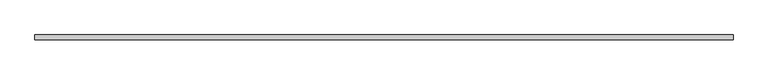
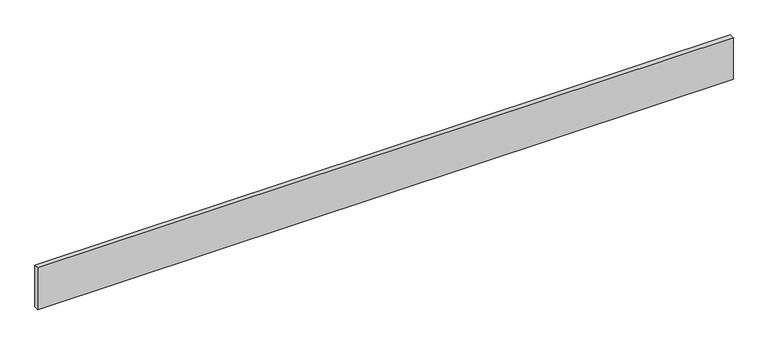
"""IFC4 building model written with IfcOpenShell, lengths in millimetres: proxy geometry, Joint001 1294 : Joint001 1294."""

import ifcopenshell
import ifcopenshell.guid

model = None  # the IFC model being written
_history = None  # IfcOwnerHistory: only IFC2X3 demands one
_inside = {}  # id of a spatial element -> (the spatial element, [elements in it])
_under = {}  # id of a project, library or spatial element -> (it, [spatial elements below it])
_declared = {}  # id of a project -> (the project, [libraries it declares])
_typed = {}  # id of a type object -> (the type object, [elements of that type])
_made_of = {}  # id of a material, layer set ... -> (it, [elements and type objects made of it])


def new_model(schema):
    """Start an empty IFC model of exactly this schema.

    Asked for "IFC4X3", IfcOpenShell would pick the latest addendum, in which some entities
    have other attributes; the version numbers below select the first issue.
    IFC2X3 requires an IfcOwnerHistory on every rooted entity: one is made here for all.
    """
    global model, _history
    if schema == "IFC4X3":
        model = ifcopenshell.file(schema_version=(4, 3, 0, 0))
    else:
        model = ifcopenshell.file(schema=schema)
    _inside.clear()
    _under.clear()
    _declared.clear()
    _typed.clear()
    _made_of.clear()
    _history = None
    if model.schema == "IFC2X3":
        org = make("IfcOrganization", Name="unknown")
        user = make(
            "IfcPersonAndOrganization",
            ThePerson=make("IfcPerson", FamilyName="unknown"),
            TheOrganization=org,
        )
        app = make(
            "IfcApplication",
            ApplicationDeveloper=org,
            Version="unknown",
            ApplicationFullName="unknown",
            ApplicationIdentifier="unknown",
        )
        _history = make(
            "IfcOwnerHistory",
            OwningUser=user,
            OwningApplication=app,
            ChangeAction="ADDED",
            CreationDate=0,
        )
    return model


def make(cls, **values):
    """One entity of the class cls with the attributes given. An attribute that is None is left unset."""
    return model.create_entity(
        cls, **{name: value for name, value in values.items() if value is not None}
    )


def rooted(cls, **values):
    """An entity with a GlobalId (a new one), such as an element, a storey or a relation."""
    return make(cls, GlobalId=ifcopenshell.guid.new(), OwnerHistory=_history, **values)


def si_unit(unit_type, name, prefix=None):
    """IfcSIUnit, for example si_unit("LENGTHUNIT", "METRE", prefix="MILLI")."""
    return make("IfcSIUnit", UnitType=unit_type, Prefix=prefix, Name=name)


def assignment(units):
    """IfcUnitAssignment: the units of a project."""
    return None if units is None else make("IfcUnitAssignment", Units=units)


def point(xyz):
    """IfcCartesianPoint."""
    return None if xyz is None else make("IfcCartesianPoint", Coordinates=xyz)


def direction(xyz):
    """IfcDirection."""
    return None if xyz is None else make("IfcDirection", DirectionRatios=xyz)


def frame(location, z_axis=None, x_axis=None):
    """IfcAxis2Placement3D, a coordinate frame: its origin and axes. An axis left out is left unset."""
    return make(
        "IfcAxis2Placement3D",
        Location=point(location),
        Axis=direction(z_axis),
        RefDirection=direction(x_axis),
    )


def origin():
    """The frame at (0, 0, 0) with its axes left unset."""
    return frame((0.0, 0.0, 0.0))


def place(relative_to, where):
    """IfcLocalPlacement: puts the frame where relative to a parent placement (None: the world)."""
    return make(
        "IfcLocalPlacement", PlacementRelTo=relative_to, RelativePlacement=where
    )


def context(
    kind, dimensions, precision=None, world=None, true_north=None, identifier=None
):
    """IfcGeometricRepresentationContext, for example the 3D "Model" context."""
    return make(
        "IfcGeometricRepresentationContext",
        ContextIdentifier=identifier,
        ContextType=kind,
        CoordinateSpaceDimension=dimensions,
        Precision=precision,
        WorldCoordinateSystem=world,
        TrueNorth=true_north,
    )


def project(units=None, contexts=None):
    """IfcProject with its units and contexts."""
    return rooted(
        "IfcProject",
        Name="project",
        RepresentationContexts=contexts,
        UnitsInContext=assignment(units),
    )


def spatial(cls, under=None, at=None, **own):
    """A site, building, storey or space (cls), placed at a placement, below another one or the project."""
    s = rooted(cls, ObjectPlacement=at, **own)
    if under is not None:
        _under.setdefault(under.id(), (under, []))[1].append(s)
    return s


def polyline(points):
    """IfcPolyline through the points."""
    return make("IfcPolyline", Points=[point(p) for p in points])


def outline(outer, holes=None, kind="AREA"):
    """IfcArbitraryClosedProfileDef: a profile drawn as a closed curve; with holes, ...WithVoids."""
    if holes is None:
        return make("IfcArbitraryClosedProfileDef", ProfileType=kind, OuterCurve=outer)
    return make(
        "IfcArbitraryProfileDefWithVoids",
        ProfileType=kind,
        OuterCurve=outer,
        InnerCurves=holes,
    )


def extrude(swept, where, along, depth):
    """IfcExtrudedAreaSolid: the profile swept, set in the frame where, extruded along a direction by depth."""
    return make(
        "IfcExtrudedAreaSolid",
        SweptArea=swept,
        Position=where,
        ExtrudedDirection=direction(along),
        Depth=depth,
    )


def shape(context_of_items, identifier, shape_type, items):
    """IfcShapeRepresentation: the items that make up one representation, for example the "Body"."""
    return make(
        "IfcShapeRepresentation",
        ContextOfItems=context_of_items,
        RepresentationIdentifier=identifier,
        RepresentationType=shape_type,
        Items=items,
    )


def source(mapping_origin, context_of_items, identifier, shape_type, items):
    """IfcRepresentationMap: a shape defined once, which mapped items show again and again."""
    return make(
        "IfcRepresentationMap",
        MappingOrigin=mapping_origin,
        MappedRepresentation=shape(context_of_items, identifier, shape_type, items),
    )


def transform(
    local_origin,
    x_axis=None,
    y_axis=None,
    z_axis=None,
    scale=None,
    scale2=None,
    scale3=None,
    uniform=True,
):
    """IfcCartesianTransformationOperator3D, or its non-uniform kind. x_axis, y_axis, z_axis: its Axis1, 2, 3."""
    if uniform:
        return make(
            "IfcCartesianTransformationOperator3D",
            Axis1=direction(x_axis),
            Axis2=direction(y_axis),
            LocalOrigin=point(local_origin),
            Scale=scale,
            Axis3=direction(z_axis),
        )
    return make(
        "IfcCartesianTransformationOperator3DnonUniform",
        Axis1=direction(x_axis),
        Axis2=direction(y_axis),
        LocalOrigin=point(local_origin),
        Scale=scale,
        Axis3=direction(z_axis),
        Scale2=scale2,
        Scale3=scale3,
    )


def mapped(mapping_source, mapping_target):
    """IfcMappedItem: shows the shape of a source again, moved by a transform."""
    return make(
        "IfcMappedItem", MappingSource=mapping_source, MappingTarget=mapping_target
    )


def made_of(thing, what):
    """Note that an element or type object is made of a material, layer set ...; save() writes the relation."""
    if what is not None:
        _made_of.setdefault(what.id(), (what, []))[1].append(thing)
    return thing


def element(
    cls,
    number,
    at=None,
    inside=None,
    cuts=None,
    type_object=None,
    material=None,
    context=None,
    identifier="Body",
    shape_type=None,
    held_by="IfcProductDefinitionShape",
    body=None,
    shapes=None,
    **own,
):
    """One element of the class cls, such as IfcWall. Its Tag is "e" and its number.

    at: its placement. inside: the storey or other place that contains it. cuts: it is an
    opening in that element (IfcRelVoidsElement). A single representation is given by context,
    identifier, shape_type and body (its items); several are given by shapes. held_by: the class
    of the entity that holds the representations. save() writes the other relations.
    """
    e = rooted(cls, Tag="e%d" % number, ObjectPlacement=at, **own)
    if body is not None:
        shapes = [shape(context, identifier, shape_type, body)]
    if shapes is not None:
        e.Representation = make(held_by, Representations=shapes)
    if inside is not None:
        _inside.setdefault(inside.id(), (inside, []))[1].append(e)
    if cuts is not None:
        rooted(
            "IfcRelVoidsElement", RelatingBuildingElement=cuts, RelatedOpeningElement=e
        )
    if type_object is not None:
        _typed.setdefault(type_object.id(), (type_object, []))[1].append(e)
    return made_of(e, material)


def aggregate(whole, parts):
    """IfcRelAggregates: a whole, such as a stair, and the parts it consists of."""
    return rooted("IfcRelAggregates", RelatingObject=whole, RelatedObjects=parts)


def save(model, path):
    """Write the relations noted so far, then the file.

    IfcRelAggregates (storeys below a building ...), IfcRelContainedInSpatialStructure (elements
    in a storey), IfcRelDefinesByType, IfcRelAssociatesMaterial and IfcRelDeclares: one each for
    every whole, place, type object, material and project.
    """
    for whole, parts in _under.values():
        aggregate(whole, parts)
    for where, things in _inside.values():
        rooted(
            "IfcRelContainedInSpatialStructure",
            RelatedElements=things,
            RelatingStructure=where,
        )
    for kind, things in _typed.values():
        rooted("IfcRelDefinesByType", RelatedObjects=things, RelatingType=kind)
    for what, things in _made_of.values():
        rooted("IfcRelAssociatesMaterial", RelatedObjects=things, RelatingMaterial=what)
    for by, libraries in _declared.values():
        rooted("IfcRelDeclares", RelatingContext=by, RelatedDefinitions=libraries)
    model.write(path)


def generic_models_d7515e32(model_context):
    return source(origin(), model_context, "Body", "SweptSolid", [
        extrude(outline(polyline([(3694.2883192, 9730.3375834), (3694.2883192, 9744.3002787), (5694.2883192, 9744.3002787), (5694.2883192, 9730.3375834), (3694.2883192, 9730.3375834)])), frame((0.0, 0.0, 36175.6882407), z_axis=(0.0, 0.0, 1.0), x_axis=(1.0, 0.0, 0.0)), (0.0, 0.0, 1.0), 127.0),
    ])


if __name__ == "__main__":
    model = new_model("IFC4")
    model_context = context("Model", 3, world=origin())
    ifc_project = project(units=[si_unit("LENGTHUNIT", "METRE", prefix="MILLI")], contexts=[model_context])
    site = spatial("IfcSite", under=ifc_project)
    building = spatial("IfcBuilding", under=site)
    placement = place(None, origin())
    generic_models_shape = generic_models_d7515e32(model_context)
    element("IfcBuildingElementProxy", 1, Name="Joint001 1294 : Joint001 1294", ObjectType="Joint001 1294 : Joint001 1294", at=placement, inside=building, context=model_context, shape_type="MappedRepresentation", body=[
        mapped(generic_models_shape, transform((0.0, 0.0, 0.0), x_axis=(1.0, 0.0, 0.0), y_axis=(0.0, 1.0, 0.0), z_axis=(0.0, 0.0, 1.0))),
    ])
    save(model, "model.ifc")

# Revit data of these elements
# Type "Joint001 1294 : Joint001 1294"
#   NameOverride = "Joint001"
# Element 1 (IfcBuildingElementProxy, "Joint001 1294 : Joint001 1294")
#   Materials on its faces: "CONCRETE EXPANSION JOINT - MINERAL FIBER"
# Materials
#   "CONCRETE EXPANSION JOINT - MINERAL FIBER": class "Unassigned", colour RGB 82 203 28, transparency 0
